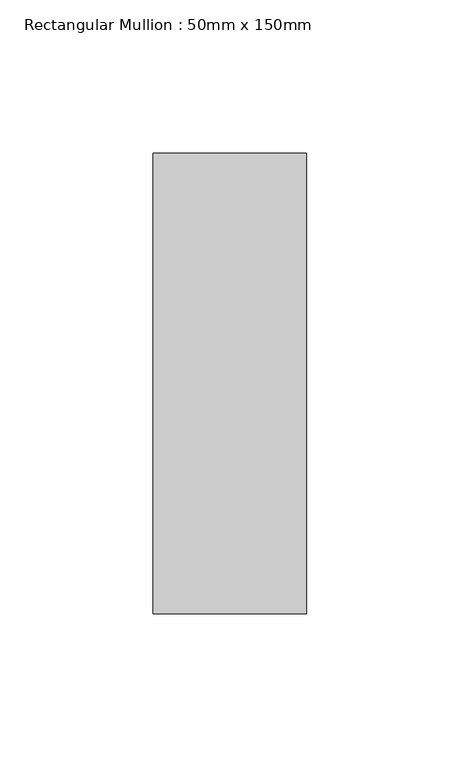
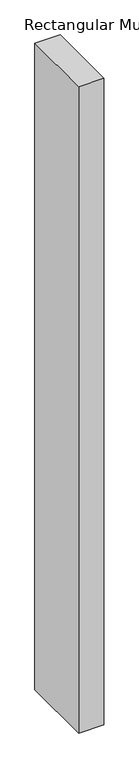
"""IFC4 building model written with IfcOpenShell, lengths in millimetres: member geometry, Rectangular Mullion : 50mm x 150mm."""

from ifc_helpers import new_model, si_unit, frame, origin, place, context, project, spatial, polyline, outline, extrude, source, transform, mapped, element, save


def rectangular_mullion_50mm_x_150mm_42f63ee8(model_context):
    return source(origin(), model_context, "Body", "SweptSolid", [
        extrude(outline(polyline([(0.0, 75.0), (0.0, -75.0), (-50.0, -75.0), (-50.0, 75.0), (0.0, 75.0)])), frame((0.0, 0.0, -1352.6802596), z_axis=(0.0, 0.0, 1.0), x_axis=(1.0, 0.0, 0.0)), (0.0, 0.0, 1.0), 1352.6802596),
    ])


if __name__ == "__main__":
    model = new_model("IFC4")
    model_context = context("Model", 3, world=origin())
    ifc_project = project(units=[si_unit("LENGTHUNIT", "METRE", prefix="MILLI")], contexts=[model_context])
    site = spatial("IfcSite", under=ifc_project)
    building = spatial("IfcBuilding", under=site)
    placement = place(None, origin())
    rectangular_mullion_50mm_x_150mm_shape = rectangular_mullion_50mm_x_150mm_42f63ee8(model_context)
    element("IfcMember", 1, ObjectType="Rectangular Mullion : 50mm x 150mm", at=placement, inside=building, context=model_context, shape_type="MappedRepresentation", body=[
        mapped(rectangular_mullion_50mm_x_150mm_shape, transform((0.0, 0.0, 0.0), x_axis=(1.0, 0.0, 0.0), y_axis=(0.0, 1.0, 0.0), z_axis=(0.0, 0.0, 1.0))),
    ])
    save(model, "model.ifc")

# Revit data of these elements
# Type "Rectangular Mullion : 50mm x 150mm"
#   built-in parameter 1007304 = 0.492126 (stored number, unit not read)
#   built-in parameter 1007301 = 0.082021 (stored number, unit not read)
#   built-in parameter 1007300 = 0.082021 (stored number, unit not read)
# Element 1 (IfcMember, "Rectangular Mullion : 50mm x 150mm")
#   Materials on its faces: "Aluminum"
# Materials
#   "Aluminum": class "Metal", colour RGB 244 244 244, transparency 0, Description = "Aluminum 6061", Cost = 0
